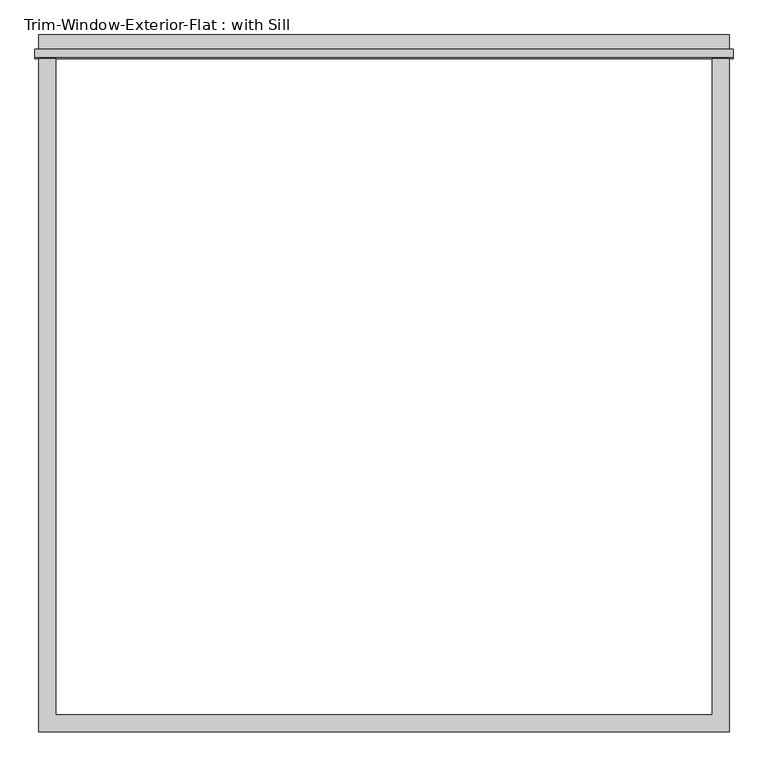
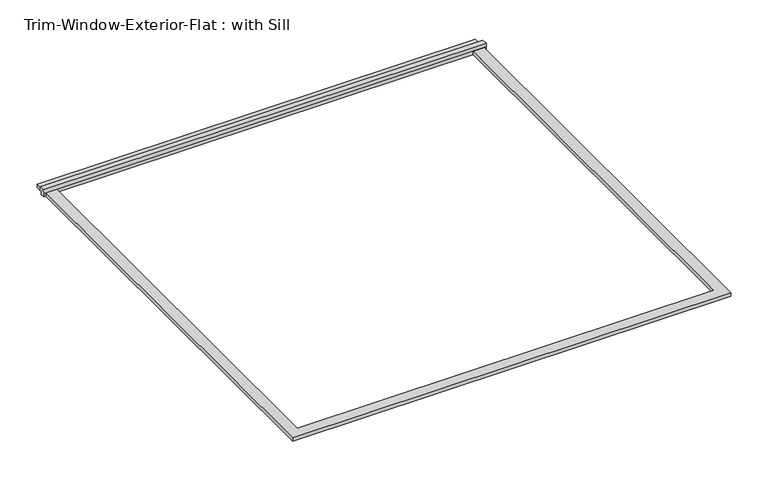
"""IFC4 building model written with IfcOpenShell, lengths in millimetres: proxy geometry, Trim-Window-Exterior-Flat : with Sill."""

from ifc_helpers import new_model, si_unit, frame, origin, origin_with_axes, place, context, project, spatial, polyline, outline, extrude, source, transform, mapped, element, save


def trim_window_exterior_flat_with_sill_f813daaf(model_context):
    return source(origin(), model_context, "Body", "SweptSolid", [
        extrude(outline(polyline([(1157.15, 2222.1823709), (-1157.15, 2222.1823709), (-1157.15, 2279.3323709), (1157.15, 2279.3323709), (1157.15, 2222.1823709)])), origin_with_axes(), (0.0, 0.0, 1.0), 19.05),
        extrude(outline(polyline([(2231.75, 38.1), (2231.75, 19.05), (2222.1823709, 19.05), (2222.1823709, 0.0), (2200.0, 0.0), (2200.0, 19.05), (2202.4580645, 38.1), (2231.75, 38.1)])), frame((-1169.85, 0.0, 0.0), z_axis=(1.0, 0.0, 0.0), x_axis=(0.0, 1.0, 0.0)), (0.0, 0.0, 1.0), 2339.7),
        extrude(outline(polyline([(-1157.15, -57.15), (-1157.15, 2200.0), (-1100.0, 2200.0), (-1100.0, 0.0), (1100.0, 0.0), (1100.0, 2200.0), (1157.15, 2200.0), (1157.15, -57.15), (-1157.15, -57.15)])), origin_with_axes(), (0.0, 0.0, 1.0), 19.05),
    ])


if __name__ == "__main__":
    model = new_model("IFC4")
    model_context = context("Model", 3, world=origin())
    ifc_project = project(units=[si_unit("LENGTHUNIT", "METRE", prefix="MILLI")], contexts=[model_context])
    site = spatial("IfcSite", under=ifc_project)
    building = spatial("IfcBuilding", under=site)
    placement = place(None, origin())
    trim_window_exterior_flat_with_sill_shape = trim_window_exterior_flat_with_sill_f813daaf(model_context)
    element("IfcBuildingElementProxy", 1, Name="Trim-Window-Exterior-Flat : with Sill", ObjectType="Trim-Window-Exterior-Flat : with Sill", at=placement, inside=building, context=model_context, shape_type="MappedRepresentation", body=[
        mapped(trim_window_exterior_flat_with_sill_shape, transform((0.0, 0.0, 0.0), x_axis=(1.0, 0.0, 0.0), y_axis=(0.0, 1.0, 0.0), z_axis=(0.0, 0.0, 1.0))),
    ])
    save(model, "model.ifc")

# Revit data of these elements
# Type "Trim-Window-Exterior-Flat : with Sill"
#   Trim Width = 0.05715 m
#   Trim Thickness_Picture Frame = 0.03175 m
#   Trim Thickness_with Sill = 0.01905 m
#   Sill Thickness = 0.03175 m
#   Opening Width [instance default] = 0.6096 m
#   Opening Height [instance default] = 0.9144 m
#   Default Elevation = 1.2192 m
#   Sill = yes
#   Picture Frame = no
#   Trim Material [instance default] = none
# Element 1 (IfcBuildingElementProxy, "Trim-Window-Exterior-Flat : with Sill")
#   Opening Width = 2.2 m
#   Opening Height = 2.2 m
#   Trim Material = Clad - White
#   Materials on its faces: "Clad - White"
# Materials
#   "Clad - White": class "Wood", colour RGB 242 242 238, transparency 0, Cost = 0
